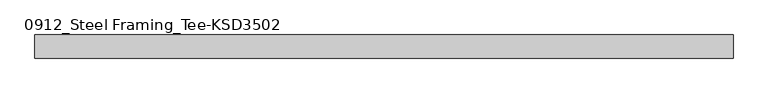
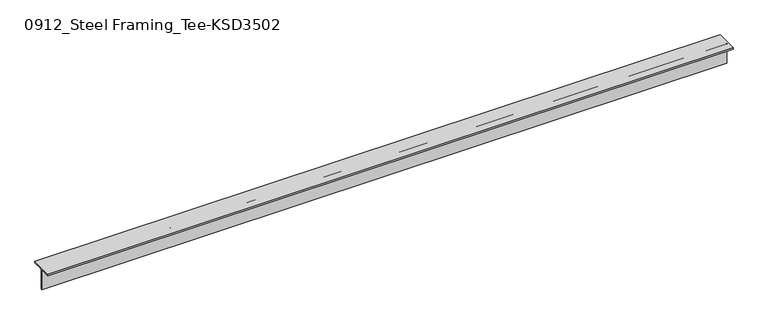
"""IFC4 building model written with IfcOpenShell, lengths in millimetres: member geometry, 0912_Steel Framing_Tee-KSD3502 : H_SB_ASB_CT-150x150x6.5x9."""

import ifcopenshell
import ifcopenshell.guid

model = None  # the IFC model being written
_history = None  # IfcOwnerHistory: only IFC2X3 demands one
_inside = {}  # id of a spatial element -> (the spatial element, [elements in it])
_under = {}  # id of a project, library or spatial element -> (it, [spatial elements below it])
_declared = {}  # id of a project -> (the project, [libraries it declares])
_typed = {}  # id of a type object -> (the type object, [elements of that type])
_made_of = {}  # id of a material, layer set ... -> (it, [elements and type objects made of it])


def new_model(schema):
    """Start an empty IFC model of exactly this schema.

    Asked for "IFC4X3", IfcOpenShell would pick the latest addendum, in which some entities
    have other attributes; the version numbers below select the first issue.
    IFC2X3 requires an IfcOwnerHistory on every rooted entity: one is made here for all.
    """
    global model, _history
    if schema == "IFC4X3":
        model = ifcopenshell.file(schema_version=(4, 3, 0, 0))
    else:
        model = ifcopenshell.file(schema=schema)
    _inside.clear()
    _under.clear()
    _declared.clear()
    _typed.clear()
    _made_of.clear()
    _history = None
    if model.schema == "IFC2X3":
        org = make("IfcOrganization", Name="unknown")
        user = make(
            "IfcPersonAndOrganization",
            ThePerson=make("IfcPerson", FamilyName="unknown"),
            TheOrganization=org,
        )
        app = make(
            "IfcApplication",
            ApplicationDeveloper=org,
            Version="unknown",
            ApplicationFullName="unknown",
            ApplicationIdentifier="unknown",
        )
        _history = make(
            "IfcOwnerHistory",
            OwningUser=user,
            OwningApplication=app,
            ChangeAction="ADDED",
            CreationDate=0,
        )
    return model


def make(cls, **values):
    """One entity of the class cls with the attributes given. An attribute that is None is left unset."""
    return model.create_entity(
        cls, **{name: value for name, value in values.items() if value is not None}
    )


def rooted(cls, **values):
    """An entity with a GlobalId (a new one), such as an element, a storey or a relation."""
    return make(cls, GlobalId=ifcopenshell.guid.new(), OwnerHistory=_history, **values)


def si_unit(unit_type, name, prefix=None):
    """IfcSIUnit, for example si_unit("LENGTHUNIT", "METRE", prefix="MILLI")."""
    return make("IfcSIUnit", UnitType=unit_type, Prefix=prefix, Name=name)


def assignment(units):
    """IfcUnitAssignment: the units of a project."""
    return None if units is None else make("IfcUnitAssignment", Units=units)


def point(xyz):
    """IfcCartesianPoint."""
    return None if xyz is None else make("IfcCartesianPoint", Coordinates=xyz)


def direction(xyz):
    """IfcDirection."""
    return None if xyz is None else make("IfcDirection", DirectionRatios=xyz)


def frame(location, z_axis=None, x_axis=None):
    """IfcAxis2Placement3D, a coordinate frame: its origin and axes. An axis left out is left unset."""
    return make(
        "IfcAxis2Placement3D",
        Location=point(location),
        Axis=direction(z_axis),
        RefDirection=direction(x_axis),
    )


def frame_2d(location, x_axis=None):
    """IfcAxis2Placement2D, a coordinate frame in the plane: its origin and x axis."""
    return make(
        "IfcAxis2Placement2D", Location=point(location), RefDirection=direction(x_axis)
    )


def origin():
    """The frame at (0, 0, 0) with its axes left unset."""
    return frame((0.0, 0.0, 0.0))


def place(relative_to, where):
    """IfcLocalPlacement: puts the frame where relative to a parent placement (None: the world)."""
    return make(
        "IfcLocalPlacement", PlacementRelTo=relative_to, RelativePlacement=where
    )


def context(
    kind, dimensions, precision=None, world=None, true_north=None, identifier=None
):
    """IfcGeometricRepresentationContext, for example the 3D "Model" context."""
    return make(
        "IfcGeometricRepresentationContext",
        ContextIdentifier=identifier,
        ContextType=kind,
        CoordinateSpaceDimension=dimensions,
        Precision=precision,
        WorldCoordinateSystem=world,
        TrueNorth=true_north,
    )


def project(units=None, contexts=None):
    """IfcProject with its units and contexts."""
    return rooted(
        "IfcProject",
        Name="project",
        RepresentationContexts=contexts,
        UnitsInContext=assignment(units),
    )


def spatial(cls, under=None, at=None, **own):
    """A site, building, storey or space (cls), placed at a placement, below another one or the project."""
    s = rooted(cls, ObjectPlacement=at, **own)
    if under is not None:
        _under.setdefault(under.id(), (under, []))[1].append(s)
    return s


def polyline(points):
    """IfcPolyline through the points."""
    return make("IfcPolyline", Points=[point(p) for p in points])


def circle_curve(where, radius):
    """IfcCircle in the frame where."""
    return make("IfcCircle", Position=where, Radius=radius)


def trimmed(basis, trim1, trim2, sense, master):
    """IfcTrimmedCurve: the piece of a basis curve between two trims."""
    return make(
        "IfcTrimmedCurve",
        BasisCurve=basis,
        Trim1=trim1,
        Trim2=trim2,
        SenseAgreement=sense,
        MasterRepresentation=master,
    )


def segment(curve, same_sense, transition):
    """IfcCompositeCurveSegment."""
    return make(
        "IfcCompositeCurveSegment",
        Transition=transition,
        SameSense=same_sense,
        ParentCurve=curve,
    )


def composite_curve(segments, self_intersect=None):
    """IfcCompositeCurve: segments joined end to end."""
    return make("IfcCompositeCurve", Segments=segments, SelfIntersect=self_intersect)


def outline(outer, holes=None, kind="AREA"):
    """IfcArbitraryClosedProfileDef: a profile drawn as a closed curve; with holes, ...WithVoids."""
    if holes is None:
        return make("IfcArbitraryClosedProfileDef", ProfileType=kind, OuterCurve=outer)
    return make(
        "IfcArbitraryProfileDefWithVoids",
        ProfileType=kind,
        OuterCurve=outer,
        InnerCurves=holes,
    )


def extrude(swept, where, along, depth):
    """IfcExtrudedAreaSolid: the profile swept, set in the frame where, extruded along a direction by depth."""
    return make(
        "IfcExtrudedAreaSolid",
        SweptArea=swept,
        Position=where,
        ExtrudedDirection=direction(along),
        Depth=depth,
    )


def shape(context_of_items, identifier, shape_type, items):
    """IfcShapeRepresentation: the items that make up one representation, for example the "Body"."""
    return make(
        "IfcShapeRepresentation",
        ContextOfItems=context_of_items,
        RepresentationIdentifier=identifier,
        RepresentationType=shape_type,
        Items=items,
    )


def source(mapping_origin, context_of_items, identifier, shape_type, items):
    """IfcRepresentationMap: a shape defined once, which mapped items show again and again."""
    return make(
        "IfcRepresentationMap",
        MappingOrigin=mapping_origin,
        MappedRepresentation=shape(context_of_items, identifier, shape_type, items),
    )


def transform(
    local_origin,
    x_axis=None,
    y_axis=None,
    z_axis=None,
    scale=None,
    scale2=None,
    scale3=None,
    uniform=True,
):
    """IfcCartesianTransformationOperator3D, or its non-uniform kind. x_axis, y_axis, z_axis: its Axis1, 2, 3."""
    if uniform:
        return make(
            "IfcCartesianTransformationOperator3D",
            Axis1=direction(x_axis),
            Axis2=direction(y_axis),
            LocalOrigin=point(local_origin),
            Scale=scale,
            Axis3=direction(z_axis),
        )
    return make(
        "IfcCartesianTransformationOperator3DnonUniform",
        Axis1=direction(x_axis),
        Axis2=direction(y_axis),
        LocalOrigin=point(local_origin),
        Scale=scale,
        Axis3=direction(z_axis),
        Scale2=scale2,
        Scale3=scale3,
    )


def mapped(mapping_source, mapping_target):
    """IfcMappedItem: shows the shape of a source again, moved by a transform."""
    return make(
        "IfcMappedItem", MappingSource=mapping_source, MappingTarget=mapping_target
    )


def made_of(thing, what):
    """Note that an element or type object is made of a material, layer set ...; save() writes the relation."""
    if what is not None:
        _made_of.setdefault(what.id(), (what, []))[1].append(thing)
    return thing


def element(
    cls,
    number,
    at=None,
    inside=None,
    cuts=None,
    type_object=None,
    material=None,
    context=None,
    identifier="Body",
    shape_type=None,
    held_by="IfcProductDefinitionShape",
    body=None,
    shapes=None,
    **own,
):
    """One element of the class cls, such as IfcWall. Its Tag is "e" and its number.

    at: its placement. inside: the storey or other place that contains it. cuts: it is an
    opening in that element (IfcRelVoidsElement). A single representation is given by context,
    identifier, shape_type and body (its items); several are given by shapes. held_by: the class
    of the entity that holds the representations. save() writes the other relations.
    """
    e = rooted(cls, Tag="e%d" % number, ObjectPlacement=at, **own)
    if body is not None:
        shapes = [shape(context, identifier, shape_type, body)]
    if shapes is not None:
        e.Representation = make(held_by, Representations=shapes)
    if inside is not None:
        _inside.setdefault(inside.id(), (inside, []))[1].append(e)
    if cuts is not None:
        rooted(
            "IfcRelVoidsElement", RelatingBuildingElement=cuts, RelatedOpeningElement=e
        )
    if type_object is not None:
        _typed.setdefault(type_object.id(), (type_object, []))[1].append(e)
    return made_of(e, material)


def aggregate(whole, parts):
    """IfcRelAggregates: a whole, such as a stair, and the parts it consists of."""
    return rooted("IfcRelAggregates", RelatingObject=whole, RelatedObjects=parts)


def save(model, path):
    """Write the relations noted so far, then the file.

    IfcRelAggregates (storeys below a building ...), IfcRelContainedInSpatialStructure (elements
    in a storey), IfcRelDefinesByType, IfcRelAssociatesMaterial and IfcRelDeclares: one each for
    every whole, place, type object, material and project.
    """
    for whole, parts in _under.values():
        aggregate(whole, parts)
    for where, things in _inside.values():
        rooted(
            "IfcRelContainedInSpatialStructure",
            RelatedElements=things,
            RelatingStructure=where,
        )
    for kind, things in _typed.values():
        rooted("IfcRelDefinesByType", RelatedObjects=things, RelatingType=kind)
    for what, things in _made_of.values():
        rooted("IfcRelAssociatesMaterial", RelatedObjects=things, RelatingMaterial=what)
    for by, libraries in _declared.values():
        rooted("IfcRelDeclares", RelatingContext=by, RelatedDefinitions=libraries)
    model.write(path)


def member_0912_steel_framing_tee_ksd3502_0b3be1fb(model_context):
    return source(origin(), model_context, "Body", "SweptSolid", [
        extrude(outline(composite_curve([segment(polyline([(-75.0, 75.0), (75.0, 75.0), (75.0, 66.0), (16.25, 66.0)]), True, "CONTINUOUS"), segment(trimmed(circle_curve(frame_2d((16.25, 53.0)), 13.0), [point((16.25, 66.0))], [point((3.25, 53.0))], True, "CARTESIAN"), True, "CONTINUOUS"), segment(polyline([(3.25, 53.0), (3.25, -75.0), (-3.25, -75.0), (-3.25, 53.0)]), True, "CONTINUOUS"), segment(trimmed(circle_curve(frame_2d((-16.25, 53.0)), 13.0), [point((-3.25, 53.0))], [point((-16.25, 66.0))], True, "CARTESIAN"), True, "CONTINUOUS"), segment(polyline([(-16.25, 66.0), (-75.0, 66.0), (-75.0, 75.0)]), True, "CONTINUOUS")], self_intersect=False)), frame((-2305.4, 0.0, 0.0), z_axis=(1.0, 0.0, 0.0), x_axis=(0.0, 1.0, 0.0)), (0.0, 0.0, 1.0), 4533.0),
    ])


if __name__ == "__main__":
    model = new_model("IFC4")
    model_context = context("Model", 3, world=origin())
    ifc_project = project(units=[si_unit("LENGTHUNIT", "METRE", prefix="MILLI")], contexts=[model_context])
    site = spatial("IfcSite", under=ifc_project)
    building = spatial("IfcBuilding", under=site)
    placement = place(None, origin())
    member_0912_steel_framing_tee_ksd3502_shape = member_0912_steel_framing_tee_ksd3502_0b3be1fb(model_context)
    element("IfcMember", 1, ObjectType="0912_Steel Framing_Tee-KSD3502 : H_SB_ASB_CT-150x150x6.5x9", at=placement, inside=building, context=model_context, shape_type="MappedRepresentation", body=[
        mapped(member_0912_steel_framing_tee_ksd3502_shape, transform((0.0, 0.0, 0.0), x_axis=(1.0, 0.0, 0.0), y_axis=(0.0, 1.0, 0.0), z_axis=(0.0, 0.0, 1.0))),
    ])
    save(model, "model.ifc")

# Revit data of these elements
# Type "0912_Steel Framing_Tee-KSD3502 : H_SB_ASB_CT-150x150x6.5x9"
#   H_WM Code_1 = "S01AA003-00001 | Main Steel Structure Fabrication Work | Shelter/Building | Light Steel - Standard (30KG/M>Weight) | Material: (   )"
#   H_WM Code_2 = "S03AA029-00001 | Main Steel Structure Erection Work | Shelter/Building | Light Steel (30KG/M>Weight) | Material: (   )"
#   H_WM Code_3 = "S01AA010-00001 | Main Steel Structure Fabrication Work | Shelter/Building | Steel Painting/Coating | for Non-Fireproofed Steel Surface, Surface Preparation, Primer, Second & Final Coat | Material: (   )"
#   H_Q'ty Cal Type Tag = "SB-Q2"
#   Width = 15.0 cm
#   Web Thickness = 0.65 cm
#   Web Fillet = 1.3 cm
#   Section Area = 23.39 cm²
#   Perimeter = 0.60 m²/m
#   Nominal Weight = 18.40 kgf/m
#   Height = 15.0 cm
#   Flange Thickness = 0.9 cm
#   Centroid Vertical = 7.5 cm
#   Centroid Horizontal = 7.5 cm
#   Length [instance default] = 1.5000 m
#   Structural Material [instance default] = Steel, 45-345
#   Warping Constant = (empty or 0)
#   Torsional Moment of Inertia = 0
#   Section Name Key = ""
#   Plastic Modulus weak axis = 0
#   Plastic Modulus strong axis = 0
#   Moment of Inertia weak axis = 0
#   Moment of Inertia strong axis = 0
#   Elastic Modulus weak axis = 0
#   Elastic Modulus strong axis = 0
#   Bolt Spacing = 0
#   Assembly Code = ""
# Element 1 (IfcMember, "0912_Steel Framing_Tee-KSD3502 : H_SB_ASB_CT-150x150x6.5x9")
#   Structural Material = none
# Materials
#   "Steel, 45-345": class "Metal", colour RGB 189 187 185, transparency 0, Description = "Steel 345 MPa", Cost = 0
